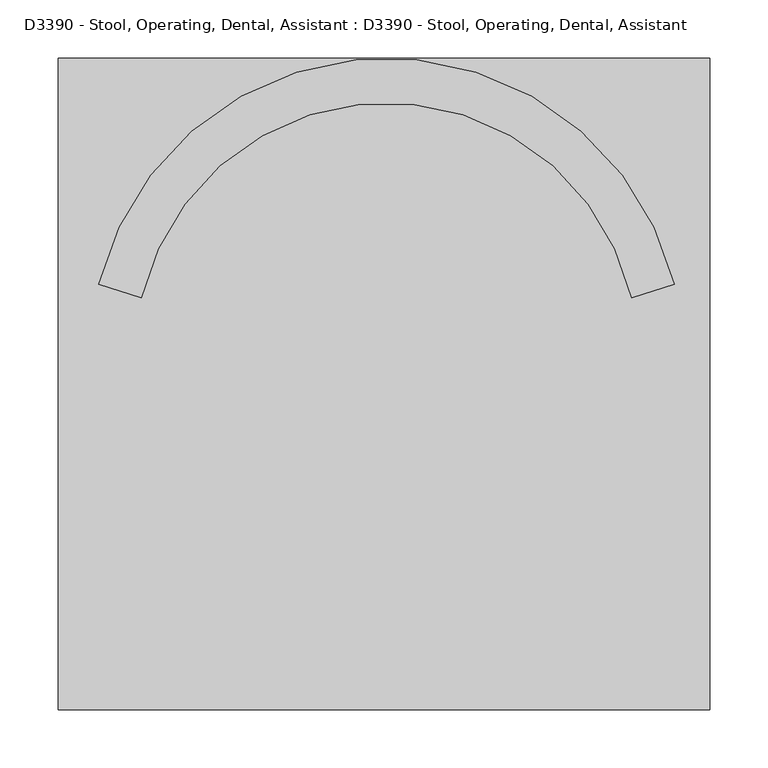
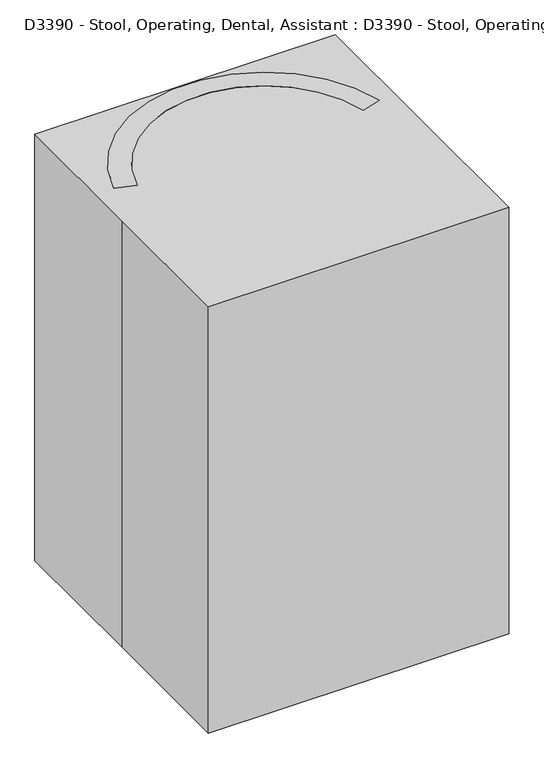
"""IFC4 building model written with IfcOpenShell, lengths in millimetres: proxy geometry, D3390 - Stool, Operating, Dental, Assistant : D3390 - Stool, Operating, Dental, Assistant."""

import ifcopenshell
import ifcopenshell.guid

model = None  # the IFC model being written
_history = None  # IfcOwnerHistory: only IFC2X3 demands one
_inside = {}  # id of a spatial element -> (the spatial element, [elements in it])
_under = {}  # id of a project, library or spatial element -> (it, [spatial elements below it])
_declared = {}  # id of a project -> (the project, [libraries it declares])
_typed = {}  # id of a type object -> (the type object, [elements of that type])
_made_of = {}  # id of a material, layer set ... -> (it, [elements and type objects made of it])


def new_model(schema):
    """Start an empty IFC model of exactly this schema.

    Asked for "IFC4X3", IfcOpenShell would pick the latest addendum, in which some entities
    have other attributes; the version numbers below select the first issue.
    IFC2X3 requires an IfcOwnerHistory on every rooted entity: one is made here for all.
    """
    global model, _history
    if schema == "IFC4X3":
        model = ifcopenshell.file(schema_version=(4, 3, 0, 0))
    else:
        model = ifcopenshell.file(schema=schema)
    _inside.clear()
    _under.clear()
    _declared.clear()
    _typed.clear()
    _made_of.clear()
    _history = None
    if model.schema == "IFC2X3":
        org = make("IfcOrganization", Name="unknown")
        user = make(
            "IfcPersonAndOrganization",
            ThePerson=make("IfcPerson", FamilyName="unknown"),
            TheOrganization=org,
        )
        app = make(
            "IfcApplication",
            ApplicationDeveloper=org,
            Version="unknown",
            ApplicationFullName="unknown",
            ApplicationIdentifier="unknown",
        )
        _history = make(
            "IfcOwnerHistory",
            OwningUser=user,
            OwningApplication=app,
            ChangeAction="ADDED",
            CreationDate=0,
        )
    return model


def make(cls, **values):
    """One entity of the class cls with the attributes given. An attribute that is None is left unset."""
    return model.create_entity(
        cls, **{name: value for name, value in values.items() if value is not None}
    )


def rooted(cls, **values):
    """An entity with a GlobalId (a new one), such as an element, a storey or a relation."""
    return make(cls, GlobalId=ifcopenshell.guid.new(), OwnerHistory=_history, **values)


def si_unit(unit_type, name, prefix=None):
    """IfcSIUnit, for example si_unit("LENGTHUNIT", "METRE", prefix="MILLI")."""
    return make("IfcSIUnit", UnitType=unit_type, Prefix=prefix, Name=name)


def assignment(units):
    """IfcUnitAssignment: the units of a project."""
    return None if units is None else make("IfcUnitAssignment", Units=units)


def point(xyz):
    """IfcCartesianPoint."""
    return None if xyz is None else make("IfcCartesianPoint", Coordinates=xyz)


def direction(xyz):
    """IfcDirection."""
    return None if xyz is None else make("IfcDirection", DirectionRatios=xyz)


def frame(location, z_axis=None, x_axis=None):
    """IfcAxis2Placement3D, a coordinate frame: its origin and axes. An axis left out is left unset."""
    return make(
        "IfcAxis2Placement3D",
        Location=point(location),
        Axis=direction(z_axis),
        RefDirection=direction(x_axis),
    )


def frame_2d(location, x_axis=None):
    """IfcAxis2Placement2D, a coordinate frame in the plane: its origin and x axis."""
    return make(
        "IfcAxis2Placement2D", Location=point(location), RefDirection=direction(x_axis)
    )


def origin():
    """The frame at (0, 0, 0) with its axes left unset."""
    return frame((0.0, 0.0, 0.0))


def origin_with_axes():
    """The frame at (0, 0, 0) with the z axis (0, 0, 1) and the x axis (1, 0, 0) written out."""
    return frame((0.0, 0.0, 0.0), z_axis=(0.0, 0.0, 1.0), x_axis=(1.0, 0.0, 0.0))


def place(relative_to, where):
    """IfcLocalPlacement: puts the frame where relative to a parent placement (None: the world)."""
    return make(
        "IfcLocalPlacement", PlacementRelTo=relative_to, RelativePlacement=where
    )


def context(
    kind, dimensions, precision=None, world=None, true_north=None, identifier=None
):
    """IfcGeometricRepresentationContext, for example the 3D "Model" context."""
    return make(
        "IfcGeometricRepresentationContext",
        ContextIdentifier=identifier,
        ContextType=kind,
        CoordinateSpaceDimension=dimensions,
        Precision=precision,
        WorldCoordinateSystem=world,
        TrueNorth=true_north,
    )


def project(units=None, contexts=None):
    """IfcProject with its units and contexts."""
    return rooted(
        "IfcProject",
        Name="project",
        RepresentationContexts=contexts,
        UnitsInContext=assignment(units),
    )


def spatial(cls, under=None, at=None, **own):
    """A site, building, storey or space (cls), placed at a placement, below another one or the project."""
    s = rooted(cls, ObjectPlacement=at, **own)
    if under is not None:
        _under.setdefault(under.id(), (under, []))[1].append(s)
    return s


def polyline(points):
    """IfcPolyline through the points."""
    return make("IfcPolyline", Points=[point(p) for p in points])


def circle_curve(where, radius):
    """IfcCircle in the frame where."""
    return make("IfcCircle", Position=where, Radius=radius)


def trimmed(basis, trim1, trim2, sense, master):
    """IfcTrimmedCurve: the piece of a basis curve between two trims."""
    return make(
        "IfcTrimmedCurve",
        BasisCurve=basis,
        Trim1=trim1,
        Trim2=trim2,
        SenseAgreement=sense,
        MasterRepresentation=master,
    )


def segment(curve, same_sense, transition):
    """IfcCompositeCurveSegment."""
    return make(
        "IfcCompositeCurveSegment",
        Transition=transition,
        SameSense=same_sense,
        ParentCurve=curve,
    )


def composite_curve(segments, self_intersect=None):
    """IfcCompositeCurve: segments joined end to end."""
    return make("IfcCompositeCurve", Segments=segments, SelfIntersect=self_intersect)


def outline(outer, holes=None, kind="AREA"):
    """IfcArbitraryClosedProfileDef: a profile drawn as a closed curve; with holes, ...WithVoids."""
    if holes is None:
        return make("IfcArbitraryClosedProfileDef", ProfileType=kind, OuterCurve=outer)
    return make(
        "IfcArbitraryProfileDefWithVoids",
        ProfileType=kind,
        OuterCurve=outer,
        InnerCurves=holes,
    )


def extrude(swept, where, along, depth):
    """IfcExtrudedAreaSolid: the profile swept, set in the frame where, extruded along a direction by depth."""
    return make(
        "IfcExtrudedAreaSolid",
        SweptArea=swept,
        Position=where,
        ExtrudedDirection=direction(along),
        Depth=depth,
    )


def shape(context_of_items, identifier, shape_type, items):
    """IfcShapeRepresentation: the items that make up one representation, for example the "Body"."""
    return make(
        "IfcShapeRepresentation",
        ContextOfItems=context_of_items,
        RepresentationIdentifier=identifier,
        RepresentationType=shape_type,
        Items=items,
    )


def source(mapping_origin, context_of_items, identifier, shape_type, items):
    """IfcRepresentationMap: a shape defined once, which mapped items show again and again."""
    return make(
        "IfcRepresentationMap",
        MappingOrigin=mapping_origin,
        MappedRepresentation=shape(context_of_items, identifier, shape_type, items),
    )


def transform(
    local_origin,
    x_axis=None,
    y_axis=None,
    z_axis=None,
    scale=None,
    scale2=None,
    scale3=None,
    uniform=True,
):
    """IfcCartesianTransformationOperator3D, or its non-uniform kind. x_axis, y_axis, z_axis: its Axis1, 2, 3."""
    if uniform:
        return make(
            "IfcCartesianTransformationOperator3D",
            Axis1=direction(x_axis),
            Axis2=direction(y_axis),
            LocalOrigin=point(local_origin),
            Scale=scale,
            Axis3=direction(z_axis),
        )
    return make(
        "IfcCartesianTransformationOperator3DnonUniform",
        Axis1=direction(x_axis),
        Axis2=direction(y_axis),
        LocalOrigin=point(local_origin),
        Scale=scale,
        Axis3=direction(z_axis),
        Scale2=scale2,
        Scale3=scale3,
    )


def mapped(mapping_source, mapping_target):
    """IfcMappedItem: shows the shape of a source again, moved by a transform."""
    return make(
        "IfcMappedItem", MappingSource=mapping_source, MappingTarget=mapping_target
    )


def made_of(thing, what):
    """Note that an element or type object is made of a material, layer set ...; save() writes the relation."""
    if what is not None:
        _made_of.setdefault(what.id(), (what, []))[1].append(thing)
    return thing


def element(
    cls,
    number,
    at=None,
    inside=None,
    cuts=None,
    type_object=None,
    material=None,
    context=None,
    identifier="Body",
    shape_type=None,
    held_by="IfcProductDefinitionShape",
    body=None,
    shapes=None,
    **own,
):
    """One element of the class cls, such as IfcWall. Its Tag is "e" and its number.

    at: its placement. inside: the storey or other place that contains it. cuts: it is an
    opening in that element (IfcRelVoidsElement). A single representation is given by context,
    identifier, shape_type and body (its items); several are given by shapes. held_by: the class
    of the entity that holds the representations. save() writes the other relations.
    """
    e = rooted(cls, Tag="e%d" % number, ObjectPlacement=at, **own)
    if body is not None:
        shapes = [shape(context, identifier, shape_type, body)]
    if shapes is not None:
        e.Representation = make(held_by, Representations=shapes)
    if inside is not None:
        _inside.setdefault(inside.id(), (inside, []))[1].append(e)
    if cuts is not None:
        rooted(
            "IfcRelVoidsElement", RelatingBuildingElement=cuts, RelatedOpeningElement=e
        )
    if type_object is not None:
        _typed.setdefault(type_object.id(), (type_object, []))[1].append(e)
    return made_of(e, material)


def aggregate(whole, parts):
    """IfcRelAggregates: a whole, such as a stair, and the parts it consists of."""
    return rooted("IfcRelAggregates", RelatingObject=whole, RelatedObjects=parts)


def save(model, path):
    """Write the relations noted so far, then the file.

    IfcRelAggregates (storeys below a building ...), IfcRelContainedInSpatialStructure (elements
    in a storey), IfcRelDefinesByType, IfcRelAssociatesMaterial and IfcRelDeclares: one each for
    every whole, place, type object, material and project.
    """
    for whole, parts in _under.values():
        aggregate(whole, parts)
    for where, things in _inside.values():
        rooted(
            "IfcRelContainedInSpatialStructure",
            RelatedElements=things,
            RelatingStructure=where,
        )
    for kind, things in _typed.values():
        rooted("IfcRelDefinesByType", RelatedObjects=things, RelatingType=kind)
    for what, things in _made_of.values():
        rooted("IfcRelAssociatesMaterial", RelatedObjects=things, RelatingMaterial=what)
    for by, libraries in _declared.values():
        rooted("IfcRelDeclares", RelatingContext=by, RelatedDefinitions=libraries)
    model.write(path)


def d3390_stool_operating_dental_assistant_d3390_stool_operating_6b55747e(model_context):
    return source(origin(), model_context, "Body", "SweptSolid", [
        extrude(outline(composite_curve([segment(polyline([(20.4732576, 248.0195063), (20.4732576, 1.7267055)]), True, "CONTINUOUS"), segment(trimmed(circle_curve(frame_2d((1.7968221, -14.3144229)), 24.6196474), [point((20.4732576, 1.7267055))], [point((-16.8796133, 1.7267055))], True, "CARTESIAN"), True, "CONTINUOUS"), segment(polyline([(-16.8796133, 1.7267055), (-16.8796133, 248.0195063), (20.4732576, 248.0195063)]), True, "CONTINUOUS")], self_intersect=False)), frame((0.0, 0.0, 444.5), z_axis=(0.0, 0.0, 1.0), x_axis=(1.0, 0.0, 0.0)), (0.0, 0.0, 1.0), 38.1),
        extrude(outline(polyline([(21.2203867, 273.4195063), (21.2203867, 248.0195063), (-16.8796133, 248.0195063), (-16.8796133, 273.4195063), (21.2203867, 273.4195063)])), frame((0.0, 0.0, 444.5), z_axis=(0.0, 0.0, 1.0), x_axis=(1.0, 0.0, 0.0)), (0.0, 0.0, 1.0), 317.5),
        extrude(outline(composite_curve([segment(polyline([(248.9451465, 85.5516246), (212.5893934, 73.7389244)]), True, "CONTINUOUS"), segment(trimmed(circle_curve(frame_2d((2.1703867, 25.4)), 215.9), [point((212.5893934, 73.7389244))], [point((-208.24862, 73.7389244))], True, "CARTESIAN"), True, "CONTINUOUS"), segment(polyline([(-208.24862, 73.7389244), (-244.604373, 85.5516246)]), True, "CONTINUOUS"), segment(trimmed(circle_curve(frame_2d((2.1703867, 25.4)), 254.0), [point((-244.604373, 85.5516246))], [point((248.9451465, 85.5516246))], False, "CARTESIAN"), True, "CONTINUOUS")], self_intersect=False)), frame((0.0, 0.0, 762.0), z_axis=(0.0, 0.0, 1.0), x_axis=(1.0, 0.0, 0.0)), (0.0, 0.0, 1.0), 76.2),
        extrude(outline(composite_curve([segment(trimmed(circle_curve(frame_2d((2.1703867, -15.1442581)), 254.0), [point((-251.8296133, -15.1442581))], [point((256.1703867, -15.1442581))], False, "CARTESIAN"), True, "CONTINUOUS"), segment(trimmed(circle_curve(frame_2d((2.1703867, -15.1442581)), 254.0), [point((256.1703867, -15.1442581))], [point((-251.8296133, -15.1442581))], False, "CARTESIAN"), True, "CONTINUOUS")], self_intersect=False)), frame((0.0, 0.0, 508.0), z_axis=(0.0, 0.0, 1.0), x_axis=(1.0, 0.0, 0.0)), (0.0, 0.0, 1.0), 50.8),
        extrude(outline(composite_curve([segment(trimmed(circle_curve(frame_2d((0.0, -25.7612183)), 25.7612183), [point((0.0, -51.5224365))], [point((0.0, 0.0))], False, "CARTESIAN"), True, "CONTINUOUS"), segment(trimmed(circle_curve(frame_2d((0.0, -25.7612183)), 25.7612183), [point((0.0, 0.0))], [point((0.0, -51.5224365))], False, "CARTESIAN"), True, "CONTINUOUS")], self_intersect=False)), frame((255.027118, 50.3219114, 25.7612183), z_axis=(-0.3090169943748919, 0.9510565162951716, 0.0), x_axis=(0.0, 0.0, 1.0)), (0.0, 0.0, 1.0), 31.75),
        extrude(outline(composite_curve([segment(polyline([(-57.1058785, 0.0), (-0.678315, 0.0)]), True, "CONTINUOUS"), segment(trimmed(circle_curve(frame_2d((-28.8920967, 0.0)), 28.2137817), [point((-0.678315, 0.0))], [point((-57.1058785, 0.0))], False, "CARTESIAN"), True, "CONTINUOUS")], self_intersect=False)), frame((258.9858893, 48.2698017, 25.7612183), z_axis=(-0.30901699437489194, 0.9510565162951717, 0.0), x_axis=(0.9510565162951717, 0.30901699437489194, 0.0)), (0.0, 0.0, 1.0), 38.1),
        extrude(outline(composite_curve([segment(trimmed(circle_curve(frame_2d((225.6213344, 57.4585541)), 3.5091751), [point((224.5369397, 60.7959779))], [point((226.7057291, 54.1211302))], False, "CARTESIAN"), True, "CONTINUOUS"), segment(trimmed(circle_curve(frame_2d((225.6213344, 57.4585541)), 3.5091751), [point((226.7057291, 54.1211302))], [point((224.5369397, 60.7959779))], False, "CARTESIAN"), True, "CONTINUOUS")], self_intersect=False)), frame((0.0, 0.0, 53.975), z_axis=(0.0, 0.0, 1.0), x_axis=(1.0, 0.0, 0.0)), (0.0, 0.0, 1.0), 13.49375),
        extrude(outline(polyline([(232.199718, 52.9196229), (27.5682802, -13.5691618), (23.6440039, -1.4914812), (228.2754417, 64.9973034), (232.199718, 52.9196229)])), frame((0.0, 0.0, 67.46875), z_axis=(0.0, 0.0, 1.0), x_axis=(1.0, 0.0, 0.0)), (0.0, 0.0, 1.0), 50.8),
        extrude(outline(composite_curve([segment(trimmed(circle_curve(frame_2d((0.0, -25.7612182)), 25.7612183), [point((0.0, -51.5224365))], [point((0.0, 0.0))], False, "CARTESIAN"), True, "CONTINUOUS"), segment(trimmed(circle_curve(frame_2d((0.0, -25.7612182)), 25.7612183), [point((0.0, 0.0))], [point((0.0, -51.5224365))], False, "CARTESIAN"), True, "CONTINUOUS")], self_intersect=False)), frame((142.5694409, -235.3951411, 25.7612183), z_axis=(0.8090169943749846, 0.5877852522924221, 0.0), x_axis=(0.0, 0.0, 1.0)), (0.0, 0.0, 1.0), 31.75),
        extrude(outline(composite_curve([segment(polyline([(-57.1058785, 0.0), (-0.6783151, 0.0)]), True, "CONTINUOUS"), segment(trimmed(circle_curve(frame_2d((-28.8920968, 0.0)), 28.2137817), [point((-0.6783151, 0.0))], [point((-57.1058785, 0.0))], False, "CARTESIAN"), True, "CONTINUOUS")], self_intersect=False)), frame((141.8410962, -239.7942932, 25.7612183), z_axis=(0.8090169943749845, 0.5877852522924221, 0.0), x_axis=(0.5877852522924221, -0.8090169943749845, 0.0)), (0.0, 0.0, 1.0), 38.1),
        extrude(outline(composite_curve([segment(trimmed(circle_curve(frame_2d((140.2699045, -205.2232351)), 3.5091751), [point((143.1088868, -203.1605938))], [point((137.4309222, -207.2858765))], False, "CARTESIAN"), True, "CONTINUOUS"), segment(trimmed(circle_curve(frame_2d((140.2699045, -205.2232351)), 3.5091751), [point((137.4309222, -207.2858765))], [point((143.1088868, -203.1605938))], False, "CARTESIAN"), True, "CONTINUOUS")], self_intersect=False)), frame((0.0, 0.0, 53.975), z_axis=(0.0, 0.0, 1.0), x_axis=(1.0, 0.0, 0.0)), (0.0, 0.0, 1.0), 13.49375),
        extrude(outline(polyline([(137.9859568, -212.8822566), (11.516773, -38.8123586), (21.7906618, -31.3479415), (148.2598455, -205.4178395), (137.9859568, -212.8822566)])), frame((0.0, 0.0, 67.46875), z_axis=(0.0, 0.0, 1.0), x_axis=(1.0, 0.0, 0.0)), (0.0, 0.0, 1.0), 50.8),
        extrude(outline(composite_curve([segment(trimmed(circle_curve(frame_2d((0.0, -25.7612183)), 25.7612183), [point((0.0, -51.5224365))], [point((0.0, 0.0))], False, "CARTESIAN"), True, "CONTINUOUS"), segment(trimmed(circle_curve(frame_2d((0.0, -25.7612183)), 25.7612183), [point((0.0, 0.0))], [point((0.0, -51.5224365))], False, "CARTESIAN"), True, "CONTINUOUS")], self_intersect=False)), frame((-138.2286675, -235.3951411, 25.7612183), z_axis=(-0.8090169943749151, 0.5877852522925178, 0.0), x_axis=(0.0, 0.0, -1.0)), (0.0, 0.0, 1.0), 31.75),
        extrude(outline(composite_curve([segment(trimmed(circle_curve(frame_2d((28.8920967, 0.0)), 28.2137817), [point((57.1058785, 0.0))], [point((0.678315, 0.0))], False, "CARTESIAN"), True, "CONTINUOUS"), segment(polyline([(0.678315, 0.0), (57.1058785, 0.0)]), True, "CONTINUOUS")], self_intersect=False)), frame((-137.5003227, -239.7942932, 25.7612183), z_axis=(-0.809016994374915, 0.5877852522925177, 0.0), x_axis=(0.5877852522925177, 0.809016994374915, 0.0)), (0.0, 0.0, 1.0), 38.1),
        extrude(outline(composite_curve([segment(trimmed(circle_curve(frame_2d((-135.9303651, -205.2223386)), 3.5091751), [point((-133.0913828, -207.28498))], [point((-138.7693474, -203.1596972))], False, "CARTESIAN"), True, "CONTINUOUS"), segment(trimmed(circle_curve(frame_2d((-135.9303651, -205.2223386)), 3.5091751), [point((-138.7693474, -203.1596972))], [point((-133.0913828, -207.28498))], False, "CARTESIAN"), True, "CONTINUOUS")], self_intersect=False)), frame((0.0, 0.0, 53.975), z_axis=(0.0, 0.0, 1.0), x_axis=(1.0, 0.0, 0.0)), (0.0, 0.0, 1.0), 13.49375),
        extrude(outline(polyline([(-143.9203061, -205.416943), (-17.4511223, -31.347045), (-7.1772336, -38.8114621), (-133.6464173, -212.88136), (-143.9203061, -205.416943)])), frame((0.0, 0.0, 67.46875), z_axis=(0.0, 0.0, 1.0), x_axis=(1.0, 0.0, 0.0)), (0.0, 0.0, 1.0), 50.8),
        extrude(outline(composite_curve([segment(trimmed(circle_curve(frame_2d((0.0, -25.7612183)), 25.7612183), [point((0.0, -51.5224365))], [point((0.0, 0.0))], False, "CARTESIAN"), True, "CONTINUOUS"), segment(trimmed(circle_curve(frame_2d((0.0, -25.7612183)), 25.7612183), [point((0.0, 0.0))], [point((0.0, -51.5224365))], False, "CARTESIAN"), True, "CONTINUOUS")], self_intersect=False)), frame((-250.6863446, 50.3219114, 25.7612183), z_axis=(0.3090169943749793, 0.9510565162951433, 0.0), x_axis=(0.0, 0.0, -1.0)), (0.0, 0.0, 1.0), 31.75),
        extrude(outline(composite_curve([segment(trimmed(circle_curve(frame_2d((28.8920968, 0.0)), 28.2137817), [point((57.1058785, 0.0))], [point((0.678315, 0.0))], False, "CARTESIAN"), True, "CONTINUOUS"), segment(polyline([(0.678315, 0.0), (57.1058785, 0.0)]), True, "CONTINUOUS")], self_intersect=False)), frame((-254.6451159, 48.2698017, 25.7612183), z_axis=(0.3090169943749793, 0.9510565162951433, 0.0), x_axis=(0.9510565162951433, -0.3090169943749793, 0.0)), (0.0, 0.0, 1.0), 38.1),
        extrude(outline(composite_curve([segment(trimmed(circle_curve(frame_2d((-221.2800896, 57.4600047)), 3.5091751), [point((-222.3644844, 54.1225809))], [point((-220.1956949, 60.7974286))], False, "CARTESIAN"), True, "CONTINUOUS"), segment(trimmed(circle_curve(frame_2d((-221.2800896, 57.4600047)), 3.5091751), [point((-220.1956949, 60.7974286))], [point((-222.3644844, 54.1225809))], False, "CARTESIAN"), True, "CONTINUOUS")], self_intersect=False)), frame((0.0, 0.0, 53.975), z_axis=(0.0, 0.0, 1.0), x_axis=(1.0, 0.0, 0.0)), (0.0, 0.0, 1.0), 13.49375),
        extrude(outline(polyline([(-223.9341969, 64.9987541), (-19.3027591, -1.4900305), (-23.2270354, -13.5677111), (-227.8584732, 52.9210735), (-223.9341969, 64.9987541)])), frame((0.0, 0.0, 67.46875), z_axis=(0.0, 0.0, 1.0), x_axis=(1.0, 0.0, 0.0)), (0.0, 0.0, 1.0), 50.8),
        extrude(outline(composite_curve([segment(trimmed(circle_curve(frame_2d((219.8057246, 25.7612183)), 25.7612183), [point((194.0445063, 25.7612183))], [point((245.5669428, 25.7612183))], False, "CARTESIAN"), True, "CONTINUOUS"), segment(trimmed(circle_curve(frame_2d((219.8057246, 25.7612183)), 25.7612183), [point((245.5669428, 25.7612183))], [point((194.0445063, 25.7612183))], False, "CARTESIAN"), True, "CONTINUOUS")], self_intersect=False)), frame((-13.7046133, 0.0, 0.0), z_axis=(1.0, 0.0, 0.0), x_axis=(0.0, 1.0, 0.0)), (0.0, 0.0, 1.0), 31.75),
        extrude(outline(composite_curve([segment(trimmed(circle_curve(frame_2d((219.8057246, 25.7612183)), 28.2137817), [point((191.5919428, 25.7612183))], [point((248.0195063, 25.7612183))], False, "CARTESIAN"), True, "CONTINUOUS"), segment(polyline([(248.0195063, 25.7612183), (191.5919428, 25.7612183)]), True, "CONTINUOUS")], self_intersect=False)), frame((-16.8796133, 0.0, 0.0), z_axis=(1.0, 0.0, 0.0), x_axis=(0.0, 1.0, 0.0)), (0.0, 0.0, 1.0), 38.1),
        extrude(outline(composite_curve([segment(trimmed(circle_curve(frame_2d((2.1711494, 219.8057246)), 3.5091751), [point((-1.3380257, 219.8057246))], [point((5.6803245, 219.8057246))], False, "CARTESIAN"), True, "CONTINUOUS"), segment(trimmed(circle_curve(frame_2d((2.1711494, 219.8057246)), 3.5091751), [point((5.6803245, 219.8057246))], [point((-1.3380257, 219.8057246))], False, "CARTESIAN"), True, "CONTINUOUS")], self_intersect=False)), frame((0.0, 0.0, 53.975), z_axis=(0.0, 0.0, 1.0), x_axis=(1.0, 0.0, 0.0)), (0.0, 0.0, 1.0), 13.49375),
        extrude(outline(polyline([(8.5207618, 224.6595323), (8.5207618, 9.4973056), (-4.178463, 9.4973056), (-4.178463, 224.6595323), (8.5207618, 224.6595323)])), frame((0.0, 0.0, 67.46875), z_axis=(0.0, 0.0, 1.0), x_axis=(1.0, 0.0, 0.0)), (0.0, 0.0, 1.0), 50.8),
        extrude(outline(composite_curve([segment(trimmed(circle_curve(frame_2d((2.1703867, -15.1442581)), 25.4466483), [point((-23.2762616, -15.1442581))], [point((27.6170351, -15.1442581))], False, "CARTESIAN"), True, "CONTINUOUS"), segment(trimmed(circle_curve(frame_2d((2.1703867, -15.1442581)), 25.4466483), [point((27.6170351, -15.1442581))], [point((-23.2762616, -15.1442581))], False, "CARTESIAN"), True, "CONTINUOUS")], self_intersect=False)), frame((0.0, 0.0, 67.46875), z_axis=(0.0, 0.0, 1.0), x_axis=(1.0, 0.0, 0.0)), (0.0, 0.0, 1.0), 440.53125),
        extrude(outline(polyline([(-279.4, 279.4), (279.4, 279.4), (279.4, -279.4), (-279.4, -279.4), (-279.4, 0.0), (-279.4, 279.4)])), origin_with_axes(), (0.0, 0.0, 1.0), 838.2),
    ])


if __name__ == "__main__":
    model = new_model("IFC4")
    model_context = context("Model", 3, world=origin())
    ifc_project = project(units=[si_unit("LENGTHUNIT", "METRE", prefix="MILLI")], contexts=[model_context])
    site = spatial("IfcSite", under=ifc_project)
    building = spatial("IfcBuilding", under=site)
    placement = place(None, origin())
    d3390_stool_operating_dental_assistant_d3390_stool_operating_shape = d3390_stool_operating_dental_assistant_d3390_stool_operating_6b55747e(model_context)
    element("IfcBuildingElementProxy", 1, Name="D3390 - Stool, Operating, Dental, Assistant : D3390 - Stool, Operating, Dental, Assistant", ObjectType="D3390 - Stool, Operating, Dental, Assistant : D3390 - Stool, Operating, Dental, Assistant", at=placement, inside=building, context=model_context, shape_type="MappedRepresentation", body=[
        mapped(d3390_stool_operating_dental_assistant_d3390_stool_operating_shape, transform((0.0, 0.0, 0.0), x_axis=(1.0, 0.0, 0.0), y_axis=(0.0, 1.0, 0.0), z_axis=(0.0, 0.0, 1.0))),
    ])
    save(model, "model.ifc")

# Revit data of these elements
# Project information
#   Room Abbreviation = "DNTP1"
#   Room Description = "Dental Treatment Room, Prosthodontic (DNTP1)"
#   Sheets - Total = "5"
#   Project Issue Date = "Issue Date"
#   Project Status = "Project Status"
#   Client Name = "Owner"
#   Project Address = "Enter address here"
#   Project Name = "Project Name"
#   Project Number = "Project Number"
#   Publication Date = "30-Jan-15"
# Type "D3390 - Stool, Operating, Dental, Assistant : D3390 - Stool, Operating, Dental, Assistant"
#   Watts2 = "0"
#   Watts1 = "0"
#   Unit_Issue = "EA"
#   UTIL_6_Misc = "-"
#   UTIL_5_NonMedGas = "-"
#   UTIL_4_MiscGas = "-"
#   UTIL_3_MedGas = "-"
#   UTIL_2_Elec = "-"
#   UTIL_1_WaterDrain = "-"
#   Nomenclature = "Stool, Operating, Dental, Assistant"
#   NSN = "6520"
#   Location [instance default] = ""
#   JSN = "D3390"
#   Fund_Source_VA = "-"
#   Fund_Source_Navy = "-"
#   Fund_Source_Army = "-"
#   Fund_Source_AF = "-"
#   ELEC_Volts2 = "0"
#   ELEC_Volts1 = "0"
#   ELEC_Phase2 = "0"
#   ELEC_Phase1 = "0"
#   ELEC_HertzSwitch = "0"
#   ELEC_HertzDependent = "0"
#   ELEC_Hertz = "0"
#   ELEC_Amps2 = "0"
#   ELEC_Amps1 = "0"
#   DetailDescription = "Dental assistant's operating stool used in dental operatories during procedures. This chair has a body support arm or abdominal support that can be left or right hand adaptable. It is also gas cylinder operated for height adjustments. The chair is available in multiple vinyl or fabric color combinations"
#   CAT_VA = "C"
#   CAT_Navy = "C"
#   CAT_IHS = "-"
#   CAT_Army = "C"
#   CAT_AF = "C"
#   BTUperhour = "0"
#   Weight_IP = 42
#   DIM_Width_IP = 1' - 10"
#   DIM_Height_IP = 2' - 9"
#   DIM_Depth_IP = 1' - 10"
# Element 1 (IfcBuildingElementProxy, "D3390 - Stool, Operating, Dental, Assistant : D3390 - Stool, Operating, Dental, Assistant")
#   Location = "DNTP1"
#   Materials on its faces: "Stool metal", "Stool caster", "Stool cushion", "EquipSpace"
# Materials
#   "Stool metal": class "Unassigned", colour RGB 201 201 201, transparency 0, Comments = "Rendering appearance not upgraded "
#   "Stool caster": class "Unassigned", colour RGB 0 0 0, transparency 0, Comments = "Rendering appearance not upgraded "
#   "Stool cushion": class "Unassigned", colour RGB 226 128 109, transparency 0, Comments = "Rendering appearance not upgraded "
#   "EquipSpace": class "Unassigned", colour RGB 221 217 195, transparency 0.5
